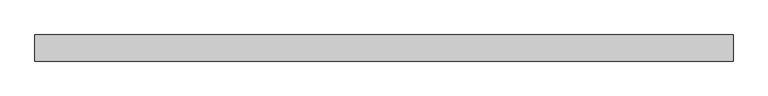
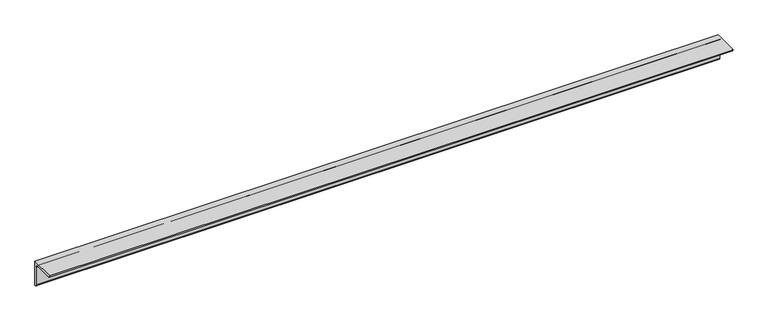
"""IFC4 building model written with IfcOpenShell, lengths in millimetres: member geometry, 0912_Steel Framing_L-KSD3502 : H_SB_AR_S03_L-130x130x12_HBR3."""

import ifcopenshell
import ifcopenshell.guid

model = None  # the IFC model being written
_history = None  # IfcOwnerHistory: only IFC2X3 demands one
_inside = {}  # id of a spatial element -> (the spatial element, [elements in it])
_under = {}  # id of a project, library or spatial element -> (it, [spatial elements below it])
_declared = {}  # id of a project -> (the project, [libraries it declares])
_typed = {}  # id of a type object -> (the type object, [elements of that type])
_made_of = {}  # id of a material, layer set ... -> (it, [elements and type objects made of it])


def new_model(schema):
    """Start an empty IFC model of exactly this schema.

    Asked for "IFC4X3", IfcOpenShell would pick the latest addendum, in which some entities
    have other attributes; the version numbers below select the first issue.
    IFC2X3 requires an IfcOwnerHistory on every rooted entity: one is made here for all.
    """
    global model, _history
    if schema == "IFC4X3":
        model = ifcopenshell.file(schema_version=(4, 3, 0, 0))
    else:
        model = ifcopenshell.file(schema=schema)
    _inside.clear()
    _under.clear()
    _declared.clear()
    _typed.clear()
    _made_of.clear()
    _history = None
    if model.schema == "IFC2X3":
        org = make("IfcOrganization", Name="unknown")
        user = make(
            "IfcPersonAndOrganization",
            ThePerson=make("IfcPerson", FamilyName="unknown"),
            TheOrganization=org,
        )
        app = make(
            "IfcApplication",
            ApplicationDeveloper=org,
            Version="unknown",
            ApplicationFullName="unknown",
            ApplicationIdentifier="unknown",
        )
        _history = make(
            "IfcOwnerHistory",
            OwningUser=user,
            OwningApplication=app,
            ChangeAction="ADDED",
            CreationDate=0,
        )
    return model


def make(cls, **values):
    """One entity of the class cls with the attributes given. An attribute that is None is left unset."""
    return model.create_entity(
        cls, **{name: value for name, value in values.items() if value is not None}
    )


def rooted(cls, **values):
    """An entity with a GlobalId (a new one), such as an element, a storey or a relation."""
    return make(cls, GlobalId=ifcopenshell.guid.new(), OwnerHistory=_history, **values)


def si_unit(unit_type, name, prefix=None):
    """IfcSIUnit, for example si_unit("LENGTHUNIT", "METRE", prefix="MILLI")."""
    return make("IfcSIUnit", UnitType=unit_type, Prefix=prefix, Name=name)


def assignment(units):
    """IfcUnitAssignment: the units of a project."""
    return None if units is None else make("IfcUnitAssignment", Units=units)


def point(xyz):
    """IfcCartesianPoint."""
    return None if xyz is None else make("IfcCartesianPoint", Coordinates=xyz)


def direction(xyz):
    """IfcDirection."""
    return None if xyz is None else make("IfcDirection", DirectionRatios=xyz)


def frame(location, z_axis=None, x_axis=None):
    """IfcAxis2Placement3D, a coordinate frame: its origin and axes. An axis left out is left unset."""
    return make(
        "IfcAxis2Placement3D",
        Location=point(location),
        Axis=direction(z_axis),
        RefDirection=direction(x_axis),
    )


def frame_2d(location, x_axis=None):
    """IfcAxis2Placement2D, a coordinate frame in the plane: its origin and x axis."""
    return make(
        "IfcAxis2Placement2D", Location=point(location), RefDirection=direction(x_axis)
    )


def origin():
    """The frame at (0, 0, 0) with its axes left unset."""
    return frame((0.0, 0.0, 0.0))


def place(relative_to, where):
    """IfcLocalPlacement: puts the frame where relative to a parent placement (None: the world)."""
    return make(
        "IfcLocalPlacement", PlacementRelTo=relative_to, RelativePlacement=where
    )


def context(
    kind, dimensions, precision=None, world=None, true_north=None, identifier=None
):
    """IfcGeometricRepresentationContext, for example the 3D "Model" context."""
    return make(
        "IfcGeometricRepresentationContext",
        ContextIdentifier=identifier,
        ContextType=kind,
        CoordinateSpaceDimension=dimensions,
        Precision=precision,
        WorldCoordinateSystem=world,
        TrueNorth=true_north,
    )


def project(units=None, contexts=None):
    """IfcProject with its units and contexts."""
    return rooted(
        "IfcProject",
        Name="project",
        RepresentationContexts=contexts,
        UnitsInContext=assignment(units),
    )


def spatial(cls, under=None, at=None, **own):
    """A site, building, storey or space (cls), placed at a placement, below another one or the project."""
    s = rooted(cls, ObjectPlacement=at, **own)
    if under is not None:
        _under.setdefault(under.id(), (under, []))[1].append(s)
    return s


def polyline(points):
    """IfcPolyline through the points."""
    return make("IfcPolyline", Points=[point(p) for p in points])


def circle_curve(where, radius):
    """IfcCircle in the frame where."""
    return make("IfcCircle", Position=where, Radius=radius)


def trimmed(basis, trim1, trim2, sense, master):
    """IfcTrimmedCurve: the piece of a basis curve between two trims."""
    return make(
        "IfcTrimmedCurve",
        BasisCurve=basis,
        Trim1=trim1,
        Trim2=trim2,
        SenseAgreement=sense,
        MasterRepresentation=master,
    )


def segment(curve, same_sense, transition):
    """IfcCompositeCurveSegment."""
    return make(
        "IfcCompositeCurveSegment",
        Transition=transition,
        SameSense=same_sense,
        ParentCurve=curve,
    )


def composite_curve(segments, self_intersect=None):
    """IfcCompositeCurve: segments joined end to end."""
    return make("IfcCompositeCurve", Segments=segments, SelfIntersect=self_intersect)


def outline(outer, holes=None, kind="AREA"):
    """IfcArbitraryClosedProfileDef: a profile drawn as a closed curve; with holes, ...WithVoids."""
    if holes is None:
        return make("IfcArbitraryClosedProfileDef", ProfileType=kind, OuterCurve=outer)
    return make(
        "IfcArbitraryProfileDefWithVoids",
        ProfileType=kind,
        OuterCurve=outer,
        InnerCurves=holes,
    )


def extrude(swept, where, along, depth):
    """IfcExtrudedAreaSolid: the profile swept, set in the frame where, extruded along a direction by depth."""
    return make(
        "IfcExtrudedAreaSolid",
        SweptArea=swept,
        Position=where,
        ExtrudedDirection=direction(along),
        Depth=depth,
    )


def shape(context_of_items, identifier, shape_type, items):
    """IfcShapeRepresentation: the items that make up one representation, for example the "Body"."""
    return make(
        "IfcShapeRepresentation",
        ContextOfItems=context_of_items,
        RepresentationIdentifier=identifier,
        RepresentationType=shape_type,
        Items=items,
    )


def source(mapping_origin, context_of_items, identifier, shape_type, items):
    """IfcRepresentationMap: a shape defined once, which mapped items show again and again."""
    return make(
        "IfcRepresentationMap",
        MappingOrigin=mapping_origin,
        MappedRepresentation=shape(context_of_items, identifier, shape_type, items),
    )


def transform(
    local_origin,
    x_axis=None,
    y_axis=None,
    z_axis=None,
    scale=None,
    scale2=None,
    scale3=None,
    uniform=True,
):
    """IfcCartesianTransformationOperator3D, or its non-uniform kind. x_axis, y_axis, z_axis: its Axis1, 2, 3."""
    if uniform:
        return make(
            "IfcCartesianTransformationOperator3D",
            Axis1=direction(x_axis),
            Axis2=direction(y_axis),
            LocalOrigin=point(local_origin),
            Scale=scale,
            Axis3=direction(z_axis),
        )
    return make(
        "IfcCartesianTransformationOperator3DnonUniform",
        Axis1=direction(x_axis),
        Axis2=direction(y_axis),
        LocalOrigin=point(local_origin),
        Scale=scale,
        Axis3=direction(z_axis),
        Scale2=scale2,
        Scale3=scale3,
    )


def mapped(mapping_source, mapping_target):
    """IfcMappedItem: shows the shape of a source again, moved by a transform."""
    return make(
        "IfcMappedItem", MappingSource=mapping_source, MappingTarget=mapping_target
    )


def made_of(thing, what):
    """Note that an element or type object is made of a material, layer set ...; save() writes the relation."""
    if what is not None:
        _made_of.setdefault(what.id(), (what, []))[1].append(thing)
    return thing


def element(
    cls,
    number,
    at=None,
    inside=None,
    cuts=None,
    type_object=None,
    material=None,
    context=None,
    identifier="Body",
    shape_type=None,
    held_by="IfcProductDefinitionShape",
    body=None,
    shapes=None,
    **own,
):
    """One element of the class cls, such as IfcWall. Its Tag is "e" and its number.

    at: its placement. inside: the storey or other place that contains it. cuts: it is an
    opening in that element (IfcRelVoidsElement). A single representation is given by context,
    identifier, shape_type and body (its items); several are given by shapes. held_by: the class
    of the entity that holds the representations. save() writes the other relations.
    """
    e = rooted(cls, Tag="e%d" % number, ObjectPlacement=at, **own)
    if body is not None:
        shapes = [shape(context, identifier, shape_type, body)]
    if shapes is not None:
        e.Representation = make(held_by, Representations=shapes)
    if inside is not None:
        _inside.setdefault(inside.id(), (inside, []))[1].append(e)
    if cuts is not None:
        rooted(
            "IfcRelVoidsElement", RelatingBuildingElement=cuts, RelatedOpeningElement=e
        )
    if type_object is not None:
        _typed.setdefault(type_object.id(), (type_object, []))[1].append(e)
    return made_of(e, material)


def aggregate(whole, parts):
    """IfcRelAggregates: a whole, such as a stair, and the parts it consists of."""
    return rooted("IfcRelAggregates", RelatingObject=whole, RelatedObjects=parts)


def save(model, path):
    """Write the relations noted so far, then the file.

    IfcRelAggregates (storeys below a building ...), IfcRelContainedInSpatialStructure (elements
    in a storey), IfcRelDefinesByType, IfcRelAssociatesMaterial and IfcRelDeclares: one each for
    every whole, place, type object, material and project.
    """
    for whole, parts in _under.values():
        aggregate(whole, parts)
    for where, things in _inside.values():
        rooted(
            "IfcRelContainedInSpatialStructure",
            RelatedElements=things,
            RelatingStructure=where,
        )
    for kind, things in _typed.values():
        rooted("IfcRelDefinesByType", RelatedObjects=things, RelatingType=kind)
    for what, things in _made_of.values():
        rooted("IfcRelAssociatesMaterial", RelatedObjects=things, RelatingMaterial=what)
    for by, libraries in _declared.values():
        rooted("IfcRelDeclares", RelatingContext=by, RelatedDefinitions=libraries)
    model.write(path)


def member_96dd18ea(model_context):
    return source(origin(), model_context, "Body", "SweptSolid", [
        extrude(outline(composite_curve([segment(polyline([(36.4, 36.4), (36.4, -93.6)]), True, "CONTINUOUS"), segment(trimmed(circle_curve(frame_2d((36.4, -81.6)), 12.0), [point((36.4, -93.6))], [point((24.4, -81.6))], False, "CARTESIAN"), True, "CONTINUOUS"), segment(polyline([(24.4, -81.6), (24.4, 12.4)]), True, "CONTINUOUS"), segment(trimmed(circle_curve(frame_2d((12.4, 12.4)), 12.0), [point((24.4, 12.4))], [point((12.4, 24.4))], True, "CARTESIAN"), True, "CONTINUOUS"), segment(polyline([(12.4, 24.4), (-81.6, 24.4)]), True, "CONTINUOUS"), segment(trimmed(circle_curve(frame_2d((-81.6, 36.4)), 12.0), [point((-81.6, 24.4))], [point((-93.6, 36.4))], False, "CARTESIAN"), True, "CONTINUOUS"), segment(polyline([(-93.6, 36.4), (36.4, 36.4)]), True, "CONTINUOUS")], self_intersect=False)), frame((-1725.9882183, 0.0, 0.0), z_axis=(1.0, 0.0, 0.0), x_axis=(0.0, 1.0, 0.0)), (0.0, 0.0, 1.0), 3476.5545794),
    ])


if __name__ == "__main__":
    model = new_model("IFC4")
    model_context = context("Model", 3, world=origin())
    ifc_project = project(units=[si_unit("LENGTHUNIT", "METRE", prefix="MILLI")], contexts=[model_context])
    site = spatial("IfcSite", under=ifc_project)
    building = spatial("IfcBuilding", under=site)
    placement = place(None, origin())
    member_shape = member_96dd18ea(model_context)
    element("IfcMember", 1, ObjectType="0912_Steel Framing_L-KSD3502 : H_SB_AR_S03_L-130x130x12_HBR3", at=placement, inside=building, context=model_context, shape_type="MappedRepresentation", body=[
        mapped(member_shape, transform((0.0, 0.0, 0.0), x_axis=(1.0, 0.0, 0.0), y_axis=(0.0, 1.0, 0.0), z_axis=(0.0, 0.0, 1.0))),
    ])
    save(model, "model.ifc")

# Revit data of these elements
# Type "0912_Steel Framing_L-KSD3502 : H_SB_AR_S03_L-130x130x12_HBR3"
#   k = 25 mm
#   Perimeter = 0.52 m²/m
#   Nominal Weight = 23.40 kgf/m
#   Length [instance default] = 1000 mm
#   b = 130 mm
#   d = 130 mm
#   t = 12 mm
#   x = 36.4 mm
#   y = 36.4 mm
#   A = 2976.00 m²
#   Structural Material [instance default] = Steel, 45-345
# Element 1 (IfcMember, "0912_Steel Framing_L-KSD3502 : H_SB_AR_S03_L-130x130x12_HBR3")
#   Materials on its faces: "Steel, 45-345"
# Materials
#   "Steel, 45-345": class "Metal", colour RGB 189 187 185, transparency 0, Description = "Steel 345 MPa", Cost = 0
